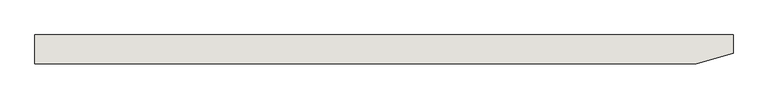
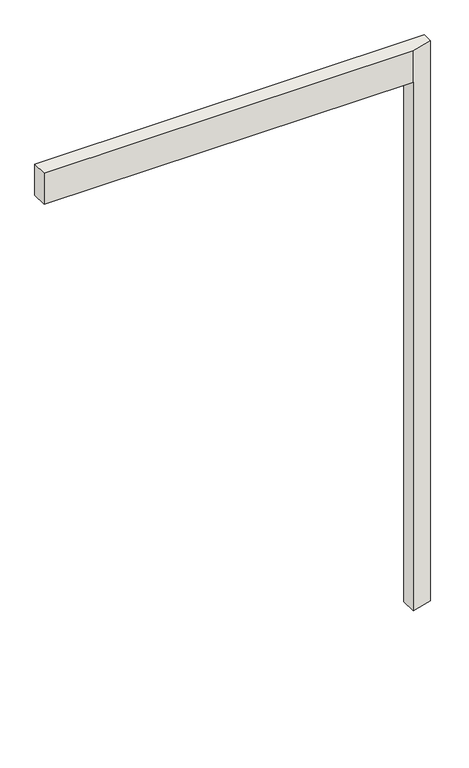
"""IFC4 building model written with IfcOpenShell, lengths in millimetres: wall geometry, 0_3d."""

from ifc_helpers import new_model, si_unit, origin, place, context, project, spatial, faceted_brep, source, transform, mapped, element, save


def wall_018feb1f(model_context):
    return source(origin(), model_context, "Body", "Brep", [
        faceted_brep([(0.0, 78.0, 2720.0), (1797.9290232, 78.0, 2720.0), (1797.9290232, 0.0, 2720.0), (0.0, 0.0, 2720.0), (1797.9290232, 78.0, 0.0), (1797.9290232, 0.0, 0.0), (0.0, 78.0, 2880.0), (1897.9290232, 78.0, 2880.0), (1897.9290232, 78.0, 0.0), (0.0, 0.0, 2880.0), (1897.9290232, 28.0, 0.0), (1897.9290232, 28.0, 2880.0), (1797.9290232, 0.0, 2880.0)], [[[0, 1, 2, 3]], [[1, 4, 5, 2]], [[4, 1, 0, 6, 7, 8]], [[0, 3, 9, 6]], [[10, 8, 7, 11]], [[5, 10, 11, 12, 2]], [[3, 2, 12, 9]], [[9, 12, 11, 7, 6]], [[5, 4, 8, 10]]]),
    ])


if __name__ == "__main__":
    model = new_model("IFC4")
    model_context = context("Model", 3, world=origin())
    ifc_project = project(units=[si_unit("LENGTHUNIT", "METRE", prefix="MILLI")], contexts=[model_context])
    site = spatial("IfcSite", under=ifc_project)
    building = spatial("IfcBuilding", under=site)
    placement = place(None, origin())
    wall_shape = wall_018feb1f(model_context)
    element("IfcWall", 1, ObjectType="0_3d", at=placement, inside=building, context=model_context, shape_type="MappedRepresentation", body=[
        mapped(wall_shape, transform((0.0, 0.0, 0.0), x_axis=(1.0, 0.0, 0.0), y_axis=(0.0, 1.0, 0.0), z_axis=(0.0, 0.0, 1.0))),
    ])
    save(model, "model.ifc")

# Revit data of these elements
# Element 1 (IfcWall, "0_3d")
#   Materials on its faces: "glas"
# Materials
#   "glas": class "Unassigned", colour RGB 250 253 254, transparency 0.95
